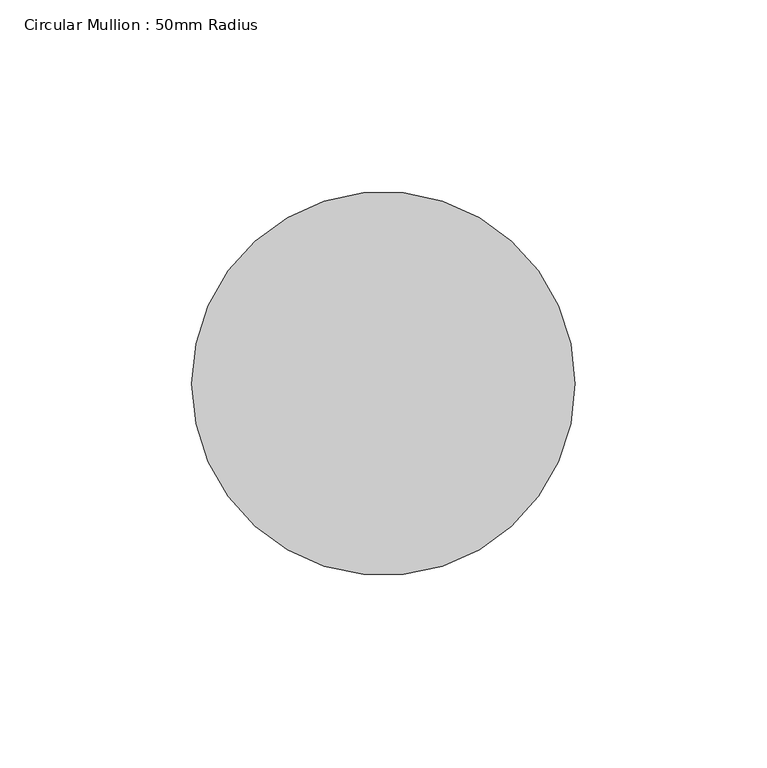
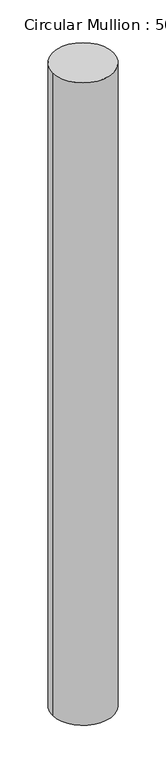
"""IFC4 building model written with IfcOpenShell, lengths in millimetres: member geometry, Circular Mullion : 50mm Radius."""

from ifc_helpers import new_model, si_unit, point, frame, origin, origin_2d, place, context, project, spatial, circle_curve, trimmed, segment, composite_curve, outline, extrude, source, transform, mapped, element, save


def circular_mullion_50mm_radius_1856102f(model_context):
    return source(origin(), model_context, "Body", "SweptSolid", [
        extrude(outline(composite_curve([segment(trimmed(circle_curve(origin_2d(), 50.0), [point((50.0, 0.0))], [point((-50.0, 0.0))], False, "CARTESIAN"), True, "CONTINUOUS"), segment(trimmed(circle_curve(origin_2d(), 50.0), [point((-50.0, 0.0))], [point((50.0, 0.0))], False, "CARTESIAN"), True, "CONTINUOUS")], self_intersect=False)), frame((0.0, 0.0, -1114.6172947), z_axis=(0.0, 0.0, 1.0), x_axis=(1.0, 0.0, 0.0)), (0.0, 0.0, 1.0), 1114.6172947),
    ])


if __name__ == "__main__":
    model = new_model("IFC4")
    model_context = context("Model", 3, world=origin())
    ifc_project = project(units=[si_unit("LENGTHUNIT", "METRE", prefix="MILLI")], contexts=[model_context])
    site = spatial("IfcSite", under=ifc_project)
    building = spatial("IfcBuilding", under=site)
    placement = place(None, origin())
    circular_mullion_50mm_radius_shape = circular_mullion_50mm_radius_1856102f(model_context)
    element("IfcMember", 1, ObjectType="Circular Mullion : 50mm Radius", at=placement, inside=building, context=model_context, shape_type="MappedRepresentation", body=[
        mapped(circular_mullion_50mm_radius_shape, transform((0.0, 0.0, 0.0), x_axis=(1.0, 0.0, 0.0), y_axis=(0.0, 1.0, 0.0), z_axis=(0.0, 0.0, 1.0))),
    ])
    save(model, "model.ifc")

# Revit data of these elements
# Type "Circular Mullion : 50mm Radius"
#   built-in parameter 1007350 = 0.164042 (stored number, unit not read)
# Element 1 (IfcMember, "Circular Mullion : 50mm Radius")
#   Materials on its faces: "Aluminium"
# Materials
#   "Aluminium": class "Metal", colour RGB 247 247 247, transparency 0, Description = "Aluminium 6061", Cost = 0
